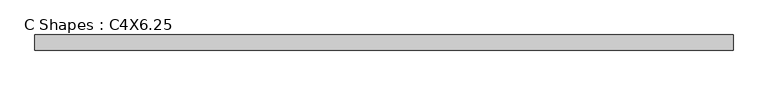
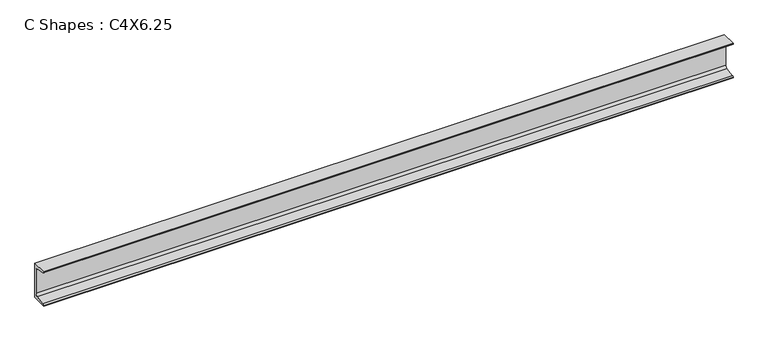
"""IFC4 building model written with IfcOpenShell, lengths in millimetres: beam geometry, C Shapes : C4X6.25."""

from ifc_helpers import new_model, si_unit, point, frame, frame_2d, origin, place, context, project, spatial, polyline, circle_curve, trimmed, segment, composite_curve, outline, extrude, source, transform, mapped, element, save


def c_shapes_c4x6_25_c3130f21(model_context):
    return source(origin(), model_context, "Body", "SweptSolid", [
        extrude(outline(composite_curve([segment(polyline([(11.049, 50.8), (11.049, -50.8), (-30.861, -50.8), (-30.861, -49.7865772)]), True, "CONTINUOUS"), segment(trimmed(circle_curve(frame_2d((-27.4066, -49.7865772)), 3.4544), [point((-30.861, -49.7865772))], [point((-27.9743618, -46.379155))], False, "CARTESIAN"), True, "CONTINUOUS"), segment(polyline([(-27.9743618, -46.379155), (-0.9980765, -41.8842311)]), True, "CONTINUOUS"), segment(trimmed(circle_curve(frame_2d((-2.1336, -35.0693868)), 6.9088), [point((-0.9980765, -41.8842311))], [point((4.7752, -35.0693868))], True, "CARTESIAN"), True, "CONTINUOUS"), segment(polyline([(4.7752, -35.0693868), (4.7752, 35.0693868)]), True, "CONTINUOUS"), segment(trimmed(circle_curve(frame_2d((-2.1336, 35.0693868)), 6.9088), [point((4.7752, 35.0693868))], [point((-0.9980765, 41.8842311))], True, "CARTESIAN"), True, "CONTINUOUS"), segment(polyline([(-0.9980765, 41.8842311), (-27.9743618, 46.379155)]), True, "CONTINUOUS"), segment(trimmed(circle_curve(frame_2d((-27.4066, 49.7865772)), 3.4544), [point((-27.9743618, 46.379155))], [point((-30.861, 49.7865772))], False, "CARTESIAN"), True, "CONTINUOUS"), segment(polyline([(-30.861, 49.7865772), (-30.861, 50.8), (11.049, 50.8)]), True, "CONTINUOUS")], self_intersect=False)), frame((-967.994, 0.0, 0.0), z_axis=(1.0, 0.0, 0.0), x_axis=(0.0, 1.0, 0.0)), (0.0, 0.0, 1.0), 1935.988),
    ])


if __name__ == "__main__":
    model = new_model("IFC4")
    model_context = context("Model", 3, world=origin())
    ifc_project = project(units=[si_unit("LENGTHUNIT", "METRE", prefix="MILLI")], contexts=[model_context])
    site = spatial("IfcSite", under=ifc_project)
    building = spatial("IfcBuilding", under=site)
    placement = place(None, origin())
    c_shapes_c4x6_25_shape = c_shapes_c4x6_25_c3130f21(model_context)
    element("IfcBeam", 1, ObjectType="C Shapes : C4X6.25", at=placement, inside=building, context=model_context, shape_type="MappedRepresentation", body=[
        mapped(c_shapes_c4x6_25_shape, transform((0.0, 0.0, 0.0), x_axis=(1.0, 0.0, 0.0), y_axis=(0.0, 1.0, 0.0), z_axis=(0.0, 0.0, 1.0))),
    ])
    save(model, "model.ifc")

# Revit data of these elements
# Type "C Shapes : C4X6.25"
#   Section Name Key = "ChannelsC4X6.25"
#   Assembly Code = "B10"
#   Width = 1.650"
#   Web Thickness = 0.247"
#   Web Fillet = 0.272"
#   Warping Constant = 1.03 in⁶
#   Torsional Moment of Inertia = 0.0487 in⁴
#   Sloped Flange Angle = 9.46°
#   Section Area = 1.77 in²
#   Plastic Modulus weak axis = 0.569 in³
#   Plastic Modulus strong axis = 2.43 in³
#   Nominal Weight = 6.25 lbf/ft
#   Moment of Inertia weak axis = 0.345 in⁴
#   Moment of Inertia strong axis = 4.00 in⁴
#   Height = 4.000"
#   Flange Thickness Location = 0.7015"
#   Flange Thickness = 0.272"
#   Flange Fillet = 0.136"
#   Elastic Modulus weak axis = 0.284 in³
#   Elastic Modulus strong axis = 2.00 in³
#   Centroid Vertical = 2.000"
#   Centroid Horizontal = 0.435"
#   Length [instance default] = 5' - 0"
#   Structural Material [instance default] = Steel ASTM A36
#   Principal Axes Angle = 0
#   Bolt Spacing = 0
# Element 1 (IfcBeam, "C Shapes : C4X6.25")
#   Materials on its faces: "Steel ASTM A36"
# Materials
#   "Steel ASTM A36": class "Metal", colour RGB 199 199 199, transparency 0, Description = "Structural steel, ASTM A36 Grade B, mill finish", Cost = 0
